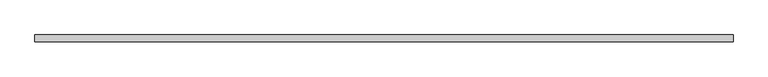
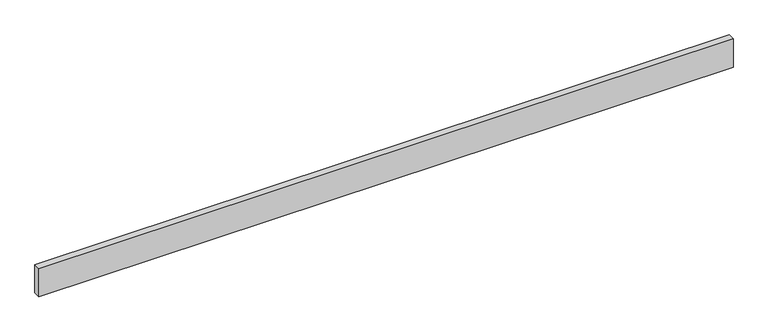
"""IFC4 building model written with IfcOpenShell, lengths in millimetres: proxy geometry, Generic Models 7:Generic Models 1:337419:Generic Models 1:337419 : Generic Models 7:Generic Models 1:337419:18 : Generic Models 7:Generic Models 1:337419:Generic Models 1:337419 : Generic Models 7:Generic Models 1:337419:301336."""

from ifc_helpers import new_model, si_unit, frame, origin, place, context, project, spatial, polyline, outline, extrude, source, transform, mapped, element, save


def generic_models_70b75125(model_context):
    return source(origin(), model_context, "Body", "SweptSolid", [
        extrude(outline(polyline([(596182.8367242, -536531.8913358), (596182.8367242, -536555.0760754), (593852.5285503, -536555.0760754), (593852.5285503, -536531.8913358), (596182.8367242, -536531.8913358)])), frame((0.0, 0.0, -23.6491575), z_axis=(0.0, 0.0, 1.0), x_axis=(1.0, 0.0, 0.0)), (0.0, 0.0, 1.0), 99.8491575),
    ])


if __name__ == "__main__":
    model = new_model("IFC4")
    model_context = context("Model", 3, world=origin())
    ifc_project = project(units=[si_unit("LENGTHUNIT", "METRE", prefix="MILLI")], contexts=[model_context])
    site = spatial("IfcSite", under=ifc_project)
    building = spatial("IfcBuilding", under=site)
    placement = place(None, origin())
    generic_models_shape = generic_models_70b75125(model_context)
    element("IfcBuildingElementProxy", 1, Name="Generic Models 7:Generic Models 1:337419:Generic Models 1:337419 : Generic Models 7:Generic Models 1:337419:18 : Generic Models 7:Generic Models 1:337419:Generic Models 1:337419 : Generic Models 7:Generic Models 1:337419:301336", ObjectType="Generic Models 7:Generic Models 1:337419:Generic Models 1:337419 : Generic Models 7:Generic Models 1:337419:18 : Generic Models 7:Generic Models 1:337419:Generic Models 1:337419 : Generic Models 7:Generic Models 1:337419:301336", at=placement, inside=building, context=model_context, shape_type="MappedRepresentation", body=[
        mapped(generic_models_shape, transform((0.0, 0.0, 0.0), x_axis=(1.0, 0.0, 0.0), y_axis=(0.0, 1.0, 0.0), z_axis=(0.0, 0.0, 1.0))),
    ])
    save(model, "model.ifc")

# Revit data of these elements
# Type "Generic Models 7:Generic Models 1:337419:Generic Models 1:337419 : Generic Models 7:Generic Models 1:337419:18 : Generic Models 7:Generic Models 1:337419:Generic Models 1:337419 : Generic Models 7:Generic Models 1:337419:301336"
#   NameOverride = "Generic Models 7:Generic Models 1:337419:Generic Models 1:337419 : Generic Models 7:Generic Models 1:337419:301336"
#   ObjectTypeOverride = "Generic Models 1:337419 : Generic Models 7:Generic Models 1:337419"
#   Reference = "Generic Models 1"
#   Tag = "301336"
# Element 1 (IfcBuildingElementProxy, "Generic Models 7:Generic Models 1:337419:Generic Models 1:337419 : Generic Models 7:Generic Models 1:337419:18 : Generic Models 7:Generic Models 1:337419:Generic Models 1:337419 : Generic Models 7:Generic Models 1:337419:301336")
#   Materials on its faces: "RIGID INSULATION AT GIRTS/JAMB - (CLASS A FLAME SPREAD)"
# Materials
#   "RIGID INSULATION AT GIRTS/JAMB - (CLASS A FLAME SPREAD)": class "Unassigned", colour RGB 205 188 106, transparency 0, Cost = 0
